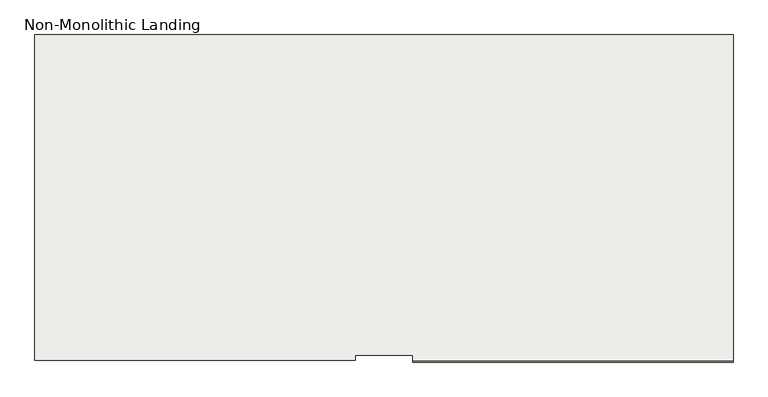
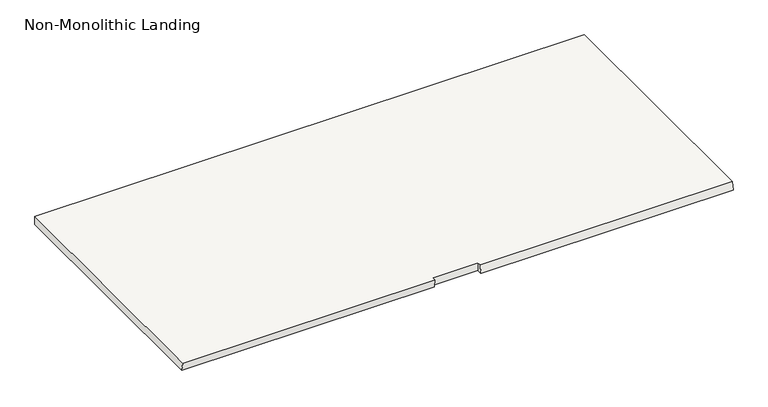
"""IFC4 building model written with IfcOpenShell, lengths in millimetres: slab geometry, Non-Monolithic Landing."""

from ifc_helpers import new_model, si_unit, origin, place, context, project, spatial, faceted_brep, source, transform, mapped, element, save


def non_monolithic_landing_f05efa27(model_context):
    return source(origin(), model_context, "Body", "Brep", [
        faceted_brep([(-226.7120949, 7307.4781803, 14617.6470588), (-226.7120949, 7300.3948469, 14567.6470588), (1293.2879051, 7300.3948469, 14567.6470588), (1293.2879051, 7307.4781803, 14617.6470588), (-499.4393676, 7309.7509075, 14617.6470588), (-499.4393676, 7332.4781803, 14617.6470588), (-226.7120949, 7332.4781803, 14617.6470588), (1293.2879051, 7332.4781803, 14617.6470588), (1293.2879051, 8852.4781803, 14617.6470588), (-2019.4393676, 8852.4781803, 14617.6470588), (-2019.4393676, 7309.7509075, 14617.6470588), (-226.7120949, 7332.4781803, 14567.6470588), (-499.4393676, 7332.4781803, 14567.6470588), (-499.4393676, 7316.8342409, 14567.6470588), (-2019.4393676, 7316.8342409, 14567.6470588), (-2019.4393676, 8852.4781803, 14567.6470588), (1293.2879051, 8852.4781803, 14567.6470588), (1293.2879051, 7332.4781803, 14567.6470588)], [[[0, 1, 2, 3]], [[4, 5, 6, 0, 3, 7, 8, 9, 10]], [[11, 12, 13, 14, 15, 16, 17, 2, 1]], [[5, 4, 13, 12]], [[6, 5, 12, 11]], [[0, 6, 11, 1]], [[7, 3, 2, 17]], [[8, 7, 17, 16]], [[9, 8, 16, 15]], [[10, 9, 15, 14]], [[4, 10, 14, 13]]]),
    ])


if __name__ == "__main__":
    model = new_model("IFC4")
    model_context = context("Model", 3, world=origin())
    ifc_project = project(units=[si_unit("LENGTHUNIT", "METRE", prefix="MILLI")], contexts=[model_context])
    site = spatial("IfcSite", under=ifc_project)
    building = spatial("IfcBuilding", under=site)
    placement = place(None, origin())
    non_monolithic_landing_shape = non_monolithic_landing_f05efa27(model_context)
    element("IfcSlab", 1, ObjectType="Non-Monolithic Landing", at=placement, inside=building, context=model_context, shape_type="MappedRepresentation", body=[
        mapped(non_monolithic_landing_shape, transform((0.0, 0.0, 0.0), x_axis=(1.0, 0.0, 0.0), y_axis=(0.0, 1.0, 0.0), z_axis=(0.0, 0.0, 1.0))),
    ])
    save(model, "model.ifc")
